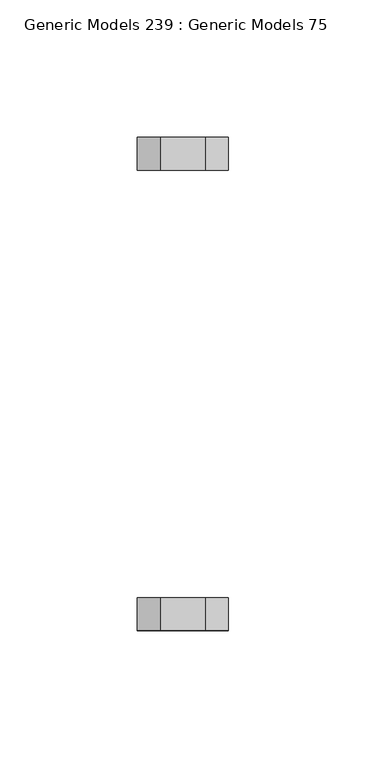
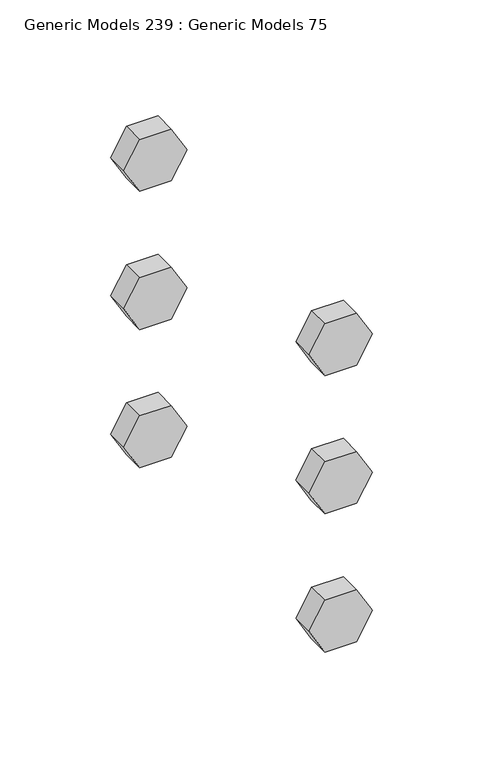
"""IFC4 building model written with IfcOpenShell, lengths in millimetres: proxy geometry, Generic Models 239 : Generic Models 75."""

from ifc_helpers import new_model, si_unit, frame, origin, place, context, project, spatial, polyline, outline, extrude, source, transform, mapped, element, save


def generic_models_239_generic_models_75_548b8a24(model_context):
    return source(origin(), model_context, "Body", "SweptSolid", [
        extrude(outline(polyline([(272027.8220065, 31971.6237939), (272013.5345065, 31979.8726858), (272013.5345065, 31996.3704698), (272027.8220065, 32004.6193618), (272042.1095065, 31996.3704698), (272042.1095065, 31979.8726858), (272027.8220065, 31971.6237939)])), frame((0.0, 36317.7270442, 0.0), z_axis=(0.0, 1.0, 0.0), x_axis=(0.0, 0.0, 1.0)), (0.0, 0.0, 1.0), 11.90625),
        extrude(outline(polyline([(272027.8220065, 31971.6237939), (272013.5345065, 31979.8726858), (272013.5345065, 31996.3704698), (272027.8220065, 32004.6193618), (272042.1095065, 31996.3704698), (272042.1095065, 31979.8726858), (272027.8220065, 31971.6237939)])), frame((0.0, 36485.2082942, 0.0), z_axis=(0.0, 1.0, 0.0), x_axis=(0.0, 0.0, 1.0)), (0.0, 0.0, 1.0), 11.90625),
        extrude(outline(polyline([(271951.6220065, 31971.6237939), (271937.3345065, 31979.8726858), (271937.3345065, 31996.3704698), (271951.6220065, 32004.6193618), (271965.9095065, 31996.3704698), (271965.9095065, 31979.8726858), (271951.6220065, 31971.6237939)])), frame((0.0, 36317.7270442, 0.0), z_axis=(0.0, 1.0, 0.0), x_axis=(0.0, 0.0, 1.0)), (0.0, 0.0, 1.0), 11.90625),
        extrude(outline(polyline([(271951.6220065, 31971.6237939), (271937.3345065, 31979.8726858), (271937.3345065, 31996.3704698), (271951.6220065, 32004.6193618), (271965.9095065, 31996.3704698), (271965.9095065, 31979.8726858), (271951.6220065, 31971.6237939)])), frame((0.0, 36485.2082942, 0.0), z_axis=(0.0, 1.0, 0.0), x_axis=(0.0, 0.0, 1.0)), (0.0, 0.0, 1.0), 11.90625),
        extrude(outline(polyline([(271875.4220065, 31971.6237939), (271861.1345065, 31979.8726858), (271861.1345065, 31996.3704698), (271875.4220065, 32004.6193618), (271889.7095065, 31996.3704698), (271889.7095065, 31979.8726858), (271875.4220065, 31971.6237939)])), frame((0.0, 36317.7270442, 0.0), z_axis=(0.0, 1.0, 0.0), x_axis=(0.0, 0.0, 1.0)), (0.0, 0.0, 1.0), 11.90625),
        extrude(outline(polyline([(271875.4220065, 31971.6237939), (271861.1345065, 31979.8726858), (271861.1345065, 31996.3704698), (271875.4220065, 32004.6193618), (271889.7095065, 31996.3704698), (271889.7095065, 31979.8726858), (271875.4220065, 31971.6237939)])), frame((0.0, 36485.2082942, 0.0), z_axis=(0.0, 1.0, 0.0), x_axis=(0.0, 0.0, 1.0)), (0.0, 0.0, 1.0), 11.90625),
    ])


if __name__ == "__main__":
    model = new_model("IFC4")
    model_context = context("Model", 3, world=origin())
    ifc_project = project(units=[si_unit("LENGTHUNIT", "METRE", prefix="MILLI")], contexts=[model_context])
    site = spatial("IfcSite", under=ifc_project)
    building = spatial("IfcBuilding", under=site)
    placement = place(None, origin())
    generic_models_239_generic_models_75_shape = generic_models_239_generic_models_75_548b8a24(model_context)
    element("IfcBuildingElementProxy", 1, Name="Generic Models 239 : Generic Models 75", ObjectType="Generic Models 239 : Generic Models 75", at=placement, inside=building, context=model_context, shape_type="MappedRepresentation", body=[
        mapped(generic_models_239_generic_models_75_shape, transform((0.0, 0.0, 0.0), x_axis=(1.0, 0.0, 0.0), y_axis=(0.0, 1.0, 0.0), z_axis=(0.0, 0.0, 1.0))),
    ])
    save(model, "model.ifc")

# Revit data of these elements
# Element 1 (IfcBuildingElementProxy, "Generic Models 239 : Generic Models 75")
#   Materials on its faces: "3/4\" GALV. THRU BOLTS"
# Materials
#   "3/4\" GALV. THRU BOLTS": class "Generic", colour RGB 105 69 171, transparency 0, Cost = 0
